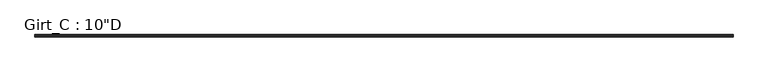
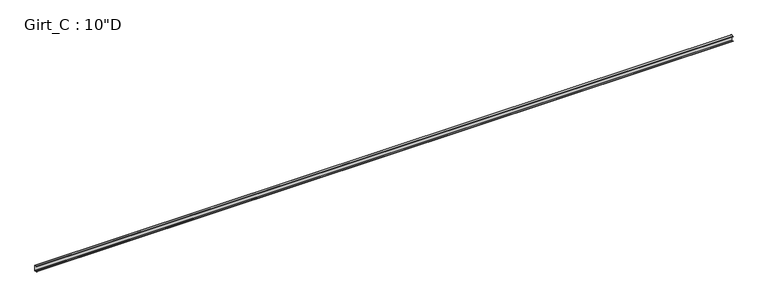
"""IFC4 building model written with IfcOpenShell, lengths in millimetres: beam geometry."""

from ifc_helpers import new_model, si_unit, point, frame, frame_2d, origin, place, context, project, spatial, polyline, circle_curve, trimmed, segment, composite_curve, outline, extrude, source, transform, mapped, element, save


def beam_8a3f25ab(model_context):
    return source(origin(), model_context, "Body", "SweptSolid", [
        extrude(outline(composite_curve([segment(polyline([(-87.5109375, 127.0), (-3.3734375, 127.0)]), True, "CONTINUOUS"), segment(trimmed(circle_curve(frame_2d((-3.3734375, 122.2375)), 4.7625), [point((-3.3734375, 127.0))], [point((1.3890625, 122.2375))], False, "CARTESIAN"), True, "CONTINUOUS"), segment(polyline([(1.3890625, 122.2375), (1.3890625, -122.2375)]), True, "CONTINUOUS"), segment(trimmed(circle_curve(frame_2d((-3.3734375, -122.2375)), 4.7625), [point((1.3890625, -122.2375))], [point((-3.3734375, -127.0))], False, "CARTESIAN"), True, "CONTINUOUS"), segment(polyline([(-3.3734375, -127.0), (-87.5109375, -127.0), (-99.7792647, -112.379177), (-97.6510975, -110.5934327), (-86.2154765, -124.221875), (-3.2694106, -124.221875)]), True, "CONTINUOUS"), segment(trimmed(circle_curve(frame_2d((-3.3748024, -122.2389339)), 1.9857399), [point((-3.2694106, -124.221875))], [point((-1.3890625, -122.2389339))], True, "CARTESIAN"), True, "CONTINUOUS"), segment(polyline([(-1.3890625, -122.2389339), (-1.3890625, 122.2381931)]), True, "CONTINUOUS"), segment(trimmed(circle_curve(frame_2d((-3.3741066, 122.2381931)), 1.9850441), [point((-1.3890625, 122.2381931))], [point((-3.3005807, 124.221875))], True, "CARTESIAN"), True, "CONTINUOUS"), segment(polyline([(-3.3005807, 124.221875), (-86.2154765, 124.221875), (-97.6278742, 110.621109), (-99.7560415, 112.4068534), (-87.5109375, 127.0)]), True, "CONTINUOUS")], self_intersect=False)), frame((-15567.025, 0.0, 0.0), z_axis=(1.0, 0.0, 0.0), x_axis=(0.0, 1.0, 0.0)), (0.0, 0.0, 1.0), 31127.7),
    ])


if __name__ == "__main__":
    model = new_model("IFC4")
    model_context = context("Model", 3, world=origin())
    ifc_project = project(units=[si_unit("LENGTHUNIT", "METRE", prefix="MILLI")], contexts=[model_context])
    site = spatial("IfcSite", under=ifc_project)
    building = spatial("IfcBuilding", under=site)
    placement = place(None, origin())
    beam_shape = beam_8a3f25ab(model_context)
    element("IfcBeam", 1, ObjectType="Girt_C : 10\"D", at=placement, inside=building, context=model_context, shape_type="MappedRepresentation", body=[
        mapped(beam_shape, transform((0.0, 0.0, 0.0), x_axis=(1.0, 0.0, 0.0), y_axis=(0.0, 1.0, 0.0), z_axis=(0.0, 0.0, 1.0))),
    ])
    save(model, "model.ifc")

# Revit data of these elements
# Type "Girt_C : 10\"D"
#   half leg = 0' - 1 3/4"
#   Web_Thickness = 0' - 0 7/64"
#   Length [instance default] = 10' - 0"
#   Leg_1 = 0' - 3 1/2"
#   Height = 0' - 10"
#   Structural Material [instance default] = none
# Element 1 (IfcBeam, "Girt_C : 10\"D")
#   Structural Material = STRUCTURAL STEEL - SEE STRUCT. DWGS
#   Materials on its faces: "STRUCTURAL STEEL - SEE STRUCT. DWGS"
# Materials
#   "STRUCTURAL STEEL - SEE STRUCT. DWGS": class "Metal", colour RGB 137 146 153, transparency 0, Description = "Steel, mill finish", Cost = 0
